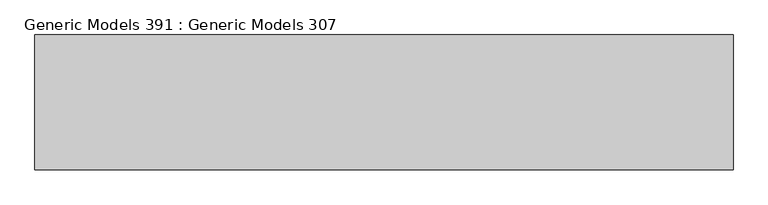
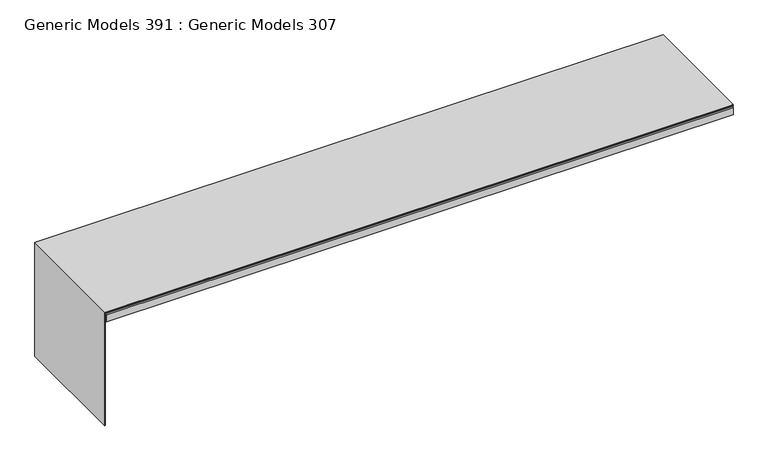
"""IFC4 building model written with IfcOpenShell, lengths in millimetres: proxy geometry, Generic Models 391 : Generic Models 307."""

from ifc_helpers import new_model, si_unit, frame, origin, place, context, project, spatial, polyline, outline, extrude, source, transform, mapped, element, save


def generic_models_391_generic_models_307_c7315f82(model_context):
    return source(origin(), model_context, "Body", "SweptSolid", [
        extrude(outline(polyline([(130157.6970742, -5562.7736296), (130158.9558462, -5562.7736296), (130158.9558462, -7140.3801921), (129857.3104462, -7140.3801921), (129857.3104462, -7139.12142), (130157.6970742, -7139.12142), (130157.6970742, -5562.7736296)])), frame((0.0, -4150.7199838, 0.0), z_axis=(0.0, 1.0, 0.0), x_axis=(0.0, 0.0, 1.0)), (0.0, 0.0, 1.0), 304.8),
        extrude(outline(polyline([(-7137.5736296, -3845.9199838), (-5562.7736296, -3845.9199838), (-5562.7736296, -4150.7199838), (-7137.5736296, -4150.7199838), (-7137.5736296, -3845.9199838)])), frame((0.0, 0.0, 130154.8791125), z_axis=(0.0, 0.0, 1.0), x_axis=(1.0, 0.0, 0.0)), (0.0, 0.0, 1.0), 1.2587721),
        extrude(outline(polyline([(-7137.5736296, -3845.9199838), (-5562.7736296, -3845.9199838), (-5562.7736296, -4150.7199838), (-7137.5736296, -4150.7199838), (-7137.5736296, -3845.9199838)])), frame((0.0, 0.0, 130131.9468019), z_axis=(0.0, 0.0, 1.0), x_axis=(1.0, 0.0, 0.0)), (0.0, 0.0, 1.0), 19.05),
    ])


if __name__ == "__main__":
    model = new_model("IFC4")
    model_context = context("Model", 3, world=origin())
    ifc_project = project(units=[si_unit("LENGTHUNIT", "METRE", prefix="MILLI")], contexts=[model_context])
    site = spatial("IfcSite", under=ifc_project)
    building = spatial("IfcBuilding", under=site)
    placement = place(None, origin())
    generic_models_391_generic_models_307_shape = generic_models_391_generic_models_307_c7315f82(model_context)
    element("IfcBuildingElementProxy", 1, Name="Generic Models 391 : Generic Models 307", ObjectType="Generic Models 391 : Generic Models 307", at=placement, inside=building, context=model_context, shape_type="MappedRepresentation", body=[
        mapped(generic_models_391_generic_models_307_shape, transform((0.0, 0.0, 0.0), x_axis=(1.0, 0.0, 0.0), y_axis=(0.0, 1.0, 0.0), z_axis=(0.0, 0.0, 1.0))),
    ])
    save(model, "model.ifc")

# Revit data of these elements
# Element 1 (IfcBuildingElementProxy, "Generic Models 391 : Generic Models 307")
#   Materials on its faces: "_(2) LAYERS NO. 30 ASTM D226 ASPHALT SATURATED ORGANIC FELT @ ROOF", "_CDX PLYWOOD - SEE STRUCT DWGs"
# Materials
#   "_(2) LAYERS NO. 30 ASTM D226 ASPHALT SATURATED ORGANIC FELT @ ROOF": class "Generic", colour RGB 67 154 161, transparency 0, Cost = 0
#   "_CDX PLYWOOD - SEE STRUCT DWGs": class "Generic", colour RGB 98 75 74, transparency 0, Cost = 0
